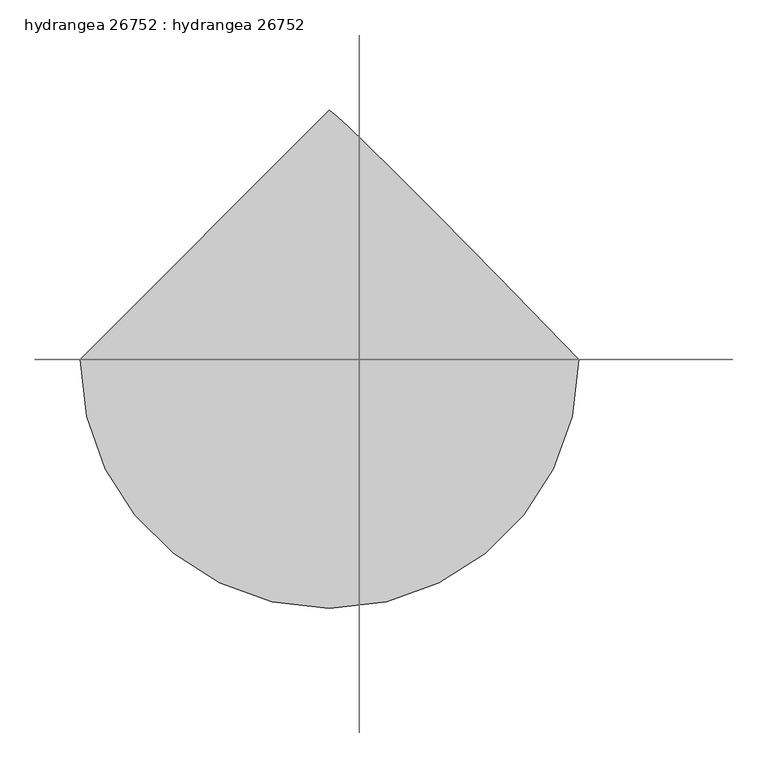
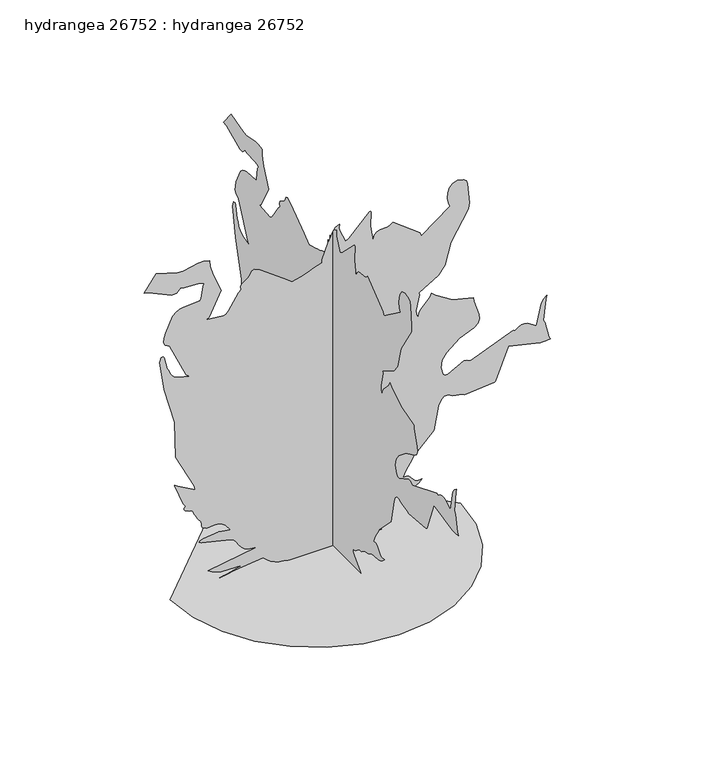
"""IFC4 building model written with IfcOpenShell, lengths in millimetres: proxy geometry, hydrangea 26752 : hydrangea 26752."""

from ifc_helpers import new_model, si_unit, origin, place, context, project, spatial, triangles, source, transform, mapped, element, save


def hydrangea_26752_hydrangea_26752_6cd4de68(model_context):
    return source(origin(), model_context, "Body", "Tessellation", [
        triangles([(-464.7672343, 0.0, 3.02e-05), (-452.4787039, -106.4936905, 3.02e-05), (-417.4875984, -204.2914365, 3.02e-05), (-362.5905132, -290.5916013, 3.02e-05), (-290.5916013, -362.5905132, 3.02e-05), (-204.2911822, -417.4875984, 3.02e-05), (-106.4936905, -452.4787039, 3.02e-05), (2.03e-05, -464.7672343, 3.02e-05), (106.4939449, -452.4787039, 3.02e-05), (204.2914365, -417.4875984, 3.02e-05), (290.5916013, -362.5905132, 3.02e-05), (362.5905132, -290.5916013, 3.02e-05), (417.4875984, -204.2911822, 3.02e-05), (452.4787039, -106.4936905, 3.02e-05), (464.7672343, 4.06e-05, 3.02e-05), (313.7284884, 154.9290062, 3.02e-05), (201.7549816, 268.9964805, 3.02e-05), (122.337727, 349.0116546, 3.02e-05), (68.9646404, 401.7878663, 3.02e-05), (35.1246865, 434.1297149, 3.02e-05), (14.3067201, 452.8546257, 3.02e-05), (-6.09e-05, 464.7672343, 3.02e-05), (56.0289111, -377.7746518, 894.66276), (56.0289111, -434.8662978, 988.0256659), (56.0289111, -437.025323, 1007.8783058), (56.0289111, -431.6938534, 1074.0784075), (56.0289111, -427.5688871, 1084.5381615), (56.0289111, -420.2181004, 1091.4545998), (56.0289111, -399.2732306, 1096.0341894), (56.0289111, -384.089092, 1091.3859993), (56.0289111, -374.1170626, 1079.9991943), (56.0289111, -368.8109911, 1064.3553091), (56.0289111, -367.6197121, 1046.9435812), (56.0289111, -369.9971832, 1030.2455452), (56.0289111, -375.3946735, 1016.7479679), (56.0289111, -283.8809099, 949.5141357), (56.0289111, -278.4503729, 960.8348837), (56.0289111, -192.0161139, 1027.487138), (56.0289111, -183.512436, 1019.3997683), (56.0289111, -173.3158381, 1016.575304), (56.0289111, -151.4921339, 1016.077442), (56.0289111, -141.6905156, 1013.0776978), (56.0289111, -133.8441922, 1004.6956512), (56.0289111, -128.8665527, 988.2669302), (56.0289111, -120.2805761, 1038.0128763), (56.0289111, -121.9587531, 1087.6699471), (56.0289111, -121.3283319, 1088.8815737), (56.0289111, -120.3204537, 1089.2625824), (56.0289111, -119.0941387, 1088.975536), (56.0289111, -117.8101691, 1088.1856133), (56.0289111, -51.0174846, 1022.5290831), (56.0289111, -40.1538944, 1015.3484894), (56.0289111, -21.3923125, 1059.6105406), (56.0289111, -19.9031842, 1068.9729778), (56.0289111, -20.5441289, 1080.248089), (56.0289111, -9.1964113, 1074.4568727), (56.0289111, -0.5405762, 1063.7304199), (56.0289111, 13.2029357, 1031.7950146), (56.0289111, 15.0194446, 1031.1828426), (56.0289111, 16.1084712, 1040.5605406), (56.0289111, 15.8290449, 1030.10333), (56.0289111, 34.9326629, 980.1719301), (56.0289111, 34.6535171, 969.7147923), (56.0289111, 46.9016657, 965.6583538), (56.0289111, 59.853396, 960.979715), (56.0289111, 73.3885619, 956.0013124), (56.0289111, 87.3888065, 951.0482718), (56.0289111, 101.7342336, 946.4457911), (56.0289111, 116.3062366, 942.5138363), (56.0289111, 130.9854187, 939.5776056), (56.0289111, 158.8299491, 961.2921232), (56.0289111, 234.3038488, 1015.5618484), (56.0289111, 252.5433605, 1023.7431805), (56.0289111, 260.6957517, 1020.4259411), (56.0289111, 264.4829115, 1008.7952557), (56.0289111, 270.9573709, 1001.4368385), (56.0289111, 292.1841821, 987.7081707), (56.0289111, 295.084859, 980.1414814), (56.0289111, 293.5100641, 968.1907574), (56.0289111, 301.5567932, 960.9593674), (56.0289111, 333.5786213, 911.8103325), (56.0289111, 341.9555446, 903.575588), (56.0289111, 350.6474195, 900.6063652), (56.0289111, 405.2778059, 906.5576008), (56.0289111, 397.091387, 912.3182957), (56.0289111, 357.3022459, 989.5521715), (56.0289111, 383.3829941, 1051.2462982), (56.0289111, 392.869915, 1083.2706516), (56.0289111, 394.0713315, 1102.6610378), (56.0289111, 413.8020676, 1107.4693199), (56.0289111, 431.2518745, 1106.8977705), (56.0289111, 479.0928497, 1096.097703), (56.0289111, 496.5959965, 1097.2025774), (56.0289111, 565.8923844, 1117.6013323), (56.0289111, 605.1150993, 1065.3077946), (56.0289111, 590.4389603, 1063.2046526), (56.0289111, 515.963528, 1028.2542423), (56.0289111, 499.8980115, 1030.0398165), (56.0289111, 487.4520052, 1042.8973166), (56.0289111, 476.9008324, 1039.305748), (56.0289111, 431.2823596, 1037.8351255), (56.0289111, 421.2823886, 1035.6633831), (56.0289111, 412.7479531, 1030.7561245), (56.0289111, 416.4106656, 1023.8879391), (56.0289111, 422.1561361, 984.398489), (56.0289111, 425.8213557, 977.5278328), (56.0289111, 478.1860737, 974.7465345), (56.0289111, 490.5939646, 971.7493338), (56.0289111, 502.2144762, 965.7473019), (56.0289111, 512.7834532, 955.7015488), (56.0289111, 536.4029417, 906.3493286), (56.0289111, 540.7590348, 890.4260273), (56.0289111, 541.4473649, 876.4001392), (56.0289111, 536.9465132, 865.9378418), (56.0289111, 523.4413055, 857.3729576), (56.0289111, 470.3247439, 742.9737631), (56.0289111, 459.1462111, 734.3275612), (56.0289111, 495.4784048, 743.0092987), (56.0289111, 506.2683349, 747.8099504), (56.0289111, 515.3336246, 754.7263887), (56.0289111, 522.0366674, 764.454574), (56.0289111, 525.7400024, 777.6930828), (56.0289111, 531.1476665, 784.7339321), (56.0289111, 539.8243172, 825.0565435), (56.0289111, 543.8298866, 829.879941), (56.0289111, 550.6015663, 829.2856459), (56.0289111, 555.6434461, 813.3064613), (56.0289111, 540.8123746, 716.5628025), (56.0289111, 507.4392663, 594.6655191), (56.0289111, 503.093347, 475.8365441), (56.0289111, 444.0484045, 359.0446904), (56.0289111, 441.1045435, 344.0002235), (56.0289111, 497.2995872, 374.7622267), (56.0289111, 506.1286268, 381.752316), (56.0289111, 507.3122755, 379.8777938), (56.0289111, 479.3442879, 309.3622215), (56.0289111, 471.5769931, 298.1760402), (56.0289111, 476.8474926, 293.4109968), (56.0289111, 476.8347754, 288.7729441), (56.0289111, 473.0577893, 284.5159002), (56.0289111, 460.289201, 278.1963731), (56.0289111, 454.3303714, 276.6495199), (56.0289111, 450.6829196, 276.5250544), (56.0289111, 447.9727289, 270.8405358), (56.0289111, 445.4428688, 265.374445), (56.0289111, 442.9105016, 259.9769365), (56.0289111, 440.1901734, 254.4981467), (56.0289111, 437.1015175, 248.789756), (56.0289111, 433.4642395, 242.6990667), (56.0289111, 429.0903422, 236.0780501), (56.0289111, 423.9341526, 231.4173971), (56.0289111, 421.2519035, 226.5421133), (56.0289111, 420.2282742, 221.6594716), (56.0289111, 420.0530305, 216.9764544), (56.0289111, 419.910779, 212.7001166), (56.0289111, 418.9912857, 209.0374223), (56.0289111, 416.4817732, 206.1956808), (56.0289111, 404.3481751, 201.1304013), (56.0289111, 392.979138, 200.8065475), (56.0289111, 381.7802576, 202.325223), (56.0289111, 370.1622894, 202.7872406), (56.0289111, 357.5257424, 199.293722), (56.0289111, 343.2814084, 188.9454982), (56.0289111, 326.8374267, 168.843146), (56.0289111, 363.7335394, 174.8182537), (56.0289111, 415.2447847, 168.959745), (56.0289111, 424.7621907, 165.1799612), (56.0289111, 427.6882476, 161.3724901), (56.0289111, 422.6031655, 158.3819023), (56.0289111, 326.8374267, 135.2257031), (56.0289111, 316.3675352, 128.5444794), (56.0289111, 308.4071926, 119.1548454), (56.0289111, 301.2011826, 108.4708318), (56.0289111, 292.9842786, 97.9059425), (56.0289111, 281.9936886, 88.8741991), (56.0289111, 266.4742689, 82.7891145), (56.0289111, 244.6604659, 81.0642016), (56.0289111, 399.6745505, 54.9174055), (56.0289111, 387.1320385, 46.4490362), (56.0289111, 358.6535079, 37.4287247), (56.0289111, 291.3510571, 36.2410178), (56.0289111, 337.9144032, 23.9287606), (56.0289111, 349.4180614, 21.3156048), (56.0289111, 362.3212709, 18.4984871), (56.0289111, 355.630909, 19.454849), (56.0289111, 338.5316257, 22.4599004), (56.0289111, 314.6454383, 26.6484415), (56.0289111, 223.7308386, 37.9362155), (56.0289111, 211.5466986, 26.1533955), (56.0289111, 198.7755668, 17.3074794), (56.0289111, 185.515475, 10.9090339), (56.0289111, 171.8642371, 6.4684733), (56.0289111, 157.9193579, 3.4965937), (56.0289111, 143.7791599, 1.5035523), (56.0289111, 129.5409211, 0.0), (56.0289111, -156.3006158, 8.5e-06), (56.0289111, -151.6640893, 6.8894283), (56.0289111, -116.3057279, 38.9204668), (56.0289111, -111.4957199, 47.331436), (56.0289111, -111.590972, 55.6176853), (56.0289111, -119.3379828, 56.8782915), (56.0289111, -125.2241879, 59.5351333), (56.0289111, -130.2038621, 63.1188217), (56.0289111, -135.2315439, 67.1597133), (56.0289111, -141.2622714, 71.1881602), (56.0289111, -149.2498198, 74.7345099), (56.0289111, -160.1494906, 77.329128), (56.0289111, -168.9650681, 83.9521794), (56.0289111, -176.5355544, 87.5539036), (56.0289111, -196.7577757, 92.3169214), (56.0289111, -204.3280077, 95.9186456), (56.0289111, -213.1436033, 102.5419604), (56.0289111, -254.4092531, 106.5686224), (56.0289111, -265.3388912, 110.053257), (56.0289111, -275.7884532, 116.2788036), (56.0289111, -285.3972962, 126.1210626), (56.0289111, -270.7287694, 125.7187253), (56.0289111, -261.0386631, 129.5500684), (56.0289111, -244.0602664, 149.2523633), (56.0289111, -236.5088377, 152.8248832), (56.0289111, -225.0498715, 152.0344246), (56.0289111, -234.5898597, 172.6625532), (56.0289111, -246.2180017, 193.2690897), (56.0289111, -259.5756166, 213.3033683), (56.0289111, -323.1010995, 276.6977727), (56.0289111, -338.0566183, 354.6326777), (56.0289111, -345.6055398, 371.0131823), (56.0289111, -356.2354506, 380.7922002), (56.0289111, -370.7261358, 381.2874825), (56.0289111, -376.1719153, 376.5935466), (56.0289111, -382.951189, 373.9163844), (56.0289111, -414.431971, 368.0820022), (56.0289111, -421.1503109, 364.0103757), (56.0289111, -516.6848866, 372.087608), (56.0289111, -521.0689213, 374.2821688), (56.0289111, -561.6327971, 477.6729873), (56.0289111, -663.3141632, 454.759633), (56.0289111, -683.0017696, 454.2617709), (56.0289111, -696.6263014, 456.4588752), (56.0289111, -691.4650612, 464.9628256), (56.0289111, -679.3771362, 518.9251568), (56.0289111, -674.215896, 527.4291072), (56.0289111, -681.6479279, 594.9220805), (56.0289111, -685.4224068, 606.8042041), (56.0289111, -674.9575659, 597.7338638), (56.0289111, -667.4314991, 587.1039531), (56.0289111, -651.805418, 516.2225965), (56.0289111, -623.5224787, 533.9975653), (56.0289111, -613.96703, 536.3114865), (56.0289111, -604.0863831, 535.7831758), (56.0289111, -593.7181206, 531.7852003), (56.0289111, -582.7021142, 523.6927437), (56.0289111, -577.4646432, 527.2970295), (56.0289111, -440.4085831, 471.9960809), (56.0289111, -429.7609045, 477.805065), (56.0289111, -420.0225454, 479.0471403), (56.0289111, -367.9321567, 451.6074635), (56.0289111, -358.5290606, 450.3882792), (56.0289111, -353.3322121, 456.9262522), (56.0289111, -345.7960078, 481.3356634), (56.0289111, -350.0683125, 504.1753667), (56.0289111, -363.3880663, 525.0059266), (56.0289111, -406.1337856, 558.9200629), (56.0289111, -451.9579871, 579.6160017), (56.0289111, -465.1685543, 589.0190978), (56.0289111, -469.6389573, 603.0043633), (56.0289111, -467.9142806, 619.826774), (56.0289111, -451.0918336, 669.8597666), (56.0289111, -450.0987256, 680.5760456), (56.0289111, -383.0096157, 698.4017744), (56.0289111, -329.3240845, 731.7240864), (56.0289111, -316.5631265, 743.6087534), (56.0289111, -311.5136164, 731.6199503), (56.0289111, -280.6932047, 700.0375757), (56.0289111, -275.2499687, 690.0807707), (56.0289111, -272.6744173, 676.8397184), (56.0289111, -266.9721128, 689.0418806), (56.0289111, -265.8748323, 702.5623489), (56.0289111, -277.0838502, 752.2879475), (56.0289111, -276.1770741, 759.2500952), (56.0289111, -338.0413939, 796.367161), (56.0289111, -358.8363819, 823.4360029), (433.8020459, 5.25e-05, 894.66276), (490.8936919, 6.21e-05, 988.0256659), (493.0552242, 6.39e-05, 1007.8783058), (487.7237909, 6.93e-05, 1074.0784075), (483.5988247, 7.01e-05, 1084.5381615), (476.2454945, 7.04e-05, 1091.4545998), (455.3006247, 7.02e-05, 1096.0341894), (440.1164861, 6.93e-05, 1091.3859993), (430.1470001, 6.81e-05, 1079.9991943), (424.8383852, 6.66e-05, 1064.3553091), (423.6496496, 6.51e-05, 1046.9435812), (426.0270844, 6.37e-05, 1030.2455452), (431.4246111, 6.27e-05, 1016.7479679), (339.9082858, 5.44e-05, 949.5141357), (334.477767, 5.52e-05, 960.8348837), (248.0447615, 5.82e-05, 1027.487138), (239.541338, 5.73e-05, 1019.3997683), (229.3447583, 5.67e-05, 1016.575304), (207.5210541, 5.6e-05, 1016.077442), (197.7191814, 5.55e-05, 1013.0776978), (189.8731124, 5.45e-05, 1004.6956512), (184.8952004, 5.3e-05, 988.2669302), (176.3092419, 5.66e-05, 1038.0128763), (177.9874098, 6.11e-05, 1087.6699471), (177.3572339, 6.11e-05, 1088.8815737), (176.3491196, 6.1e-05, 1089.2625824), (175.1227954, 6.09e-05, 1088.975536), (173.8390802, 6.07e-05, 1088.1856133), (107.0464002, 5.35e-05, 1022.5290831), (96.182801, 5.27e-05, 1015.3484894), (77.4210737, 5.59e-05, 1059.6105406), (75.9321248, 5.66e-05, 1068.9729778), (76.5729696, 5.75e-05, 1080.248089), (65.2252475, 5.67e-05, 1074.4568727), (56.5694259, 5.55e-05, 1063.7304199), (42.8259742, 5.23e-05, 1031.7950146), (41.0093655, 5.23e-05, 1031.1828426), (39.9204648, 5.31e-05, 1040.5605406), (40.1998673, 5.22e-05, 1030.10333), (21.0960983, 4.75e-05, 980.1719301), (21.3753963, 4.66e-05, 969.7147923), (9.1270438, 4.59e-05, 965.6583538), (-3.8244574, 4.51e-05, 960.979715), (-17.3597019, 4.43e-05, 956.0013124), (-31.3598954, 4.34e-05, 951.0482718), (-45.7053225, 4.26e-05, 946.4457911), (-60.2773209, 4.18e-05, 942.5138363), (-74.9565076, 4.11e-05, 939.5776056), (-102.801038, 4.21e-05, 961.2921232), (-178.2749468, 4.45e-05, 1015.5618484), (-196.5144585, 4.46e-05, 1023.7431805), (-204.6668497, 4.41e-05, 1020.4259411), (-208.4534826, 4.3e-05, 1008.7952557), (-214.9284508, 4.22e-05, 1001.4368385), (-236.1547533, 4.05e-05, 987.7081707), (-239.055957, 3.97e-05, 980.1414814), (-237.481907, 3.88e-05, 968.1907574), (-245.5273643, 3.79e-05, 960.9593674), (-277.5486837, 3.28e-05, 911.8103325), (-285.9281505, 3.19e-05, 903.575588), (-294.6200436, 3.14e-05, 900.6063652), (-349.2479047, 3.02e-05, 906.5576008), (-341.0639929, 3.09e-05, 912.3182957), (-301.2723083, 3.86e-05, 989.5521715), (-327.3530565, 4.31e-05, 1051.2462982), (-336.8399775, 4.55e-05, 1083.2706516), (-338.0413939, 4.71e-05, 1102.6610378), (-357.77213, 4.69e-05, 1107.4693199), (-375.2244804, 4.63e-05, 1106.8977705), (-423.0654556, 4.4e-05, 1096.097703), (-440.5660953, 4.36e-05, 1097.2025774), (-509.8649903, 4.32e-05, 1117.6013323), (-549.0851618, 3.76e-05, 1065.3077946), (-534.4115662, 3.79e-05, 1063.2046526), (-459.9361339, 3.72e-05, 1028.2542423), (-443.8706174, 3.78e-05, 1030.0398165), (-431.4246111, 3.93e-05, 1042.8973166), (-420.8734383, 3.93e-05, 1039.305748), (-375.252422, 4.05e-05, 1037.8351255), (-365.252451, 4.06e-05, 1035.6633831), (-356.7180519, 4.05e-05, 1030.7561245), (-360.3832715, 3.98e-05, 1023.8879391), (-366.128742, 3.63e-05, 984.398489), (-369.7914182, 3.56e-05, 977.5278328), (-422.1586796, 3.38e-05, 974.7465345), (-434.5666068, 3.32e-05, 971.7493338), (-446.184575, 3.23e-05, 965.7473019), (-456.7535156, 3.12e-05, 955.7015488), (-480.3730042, 2.63e-05, 906.3493286), (-484.7290973, 2.48e-05, 890.4260273), (-485.4174637, 2.36e-05, 876.4001392), (-480.9165756, 2.29e-05, 865.9378418), (-467.4139114, 2.25e-05, 857.3729576), (-414.2948427, 1.45e-05, 742.9737631), (-403.118817, 1.41e-05, 734.3275612), (-439.4484673, 1.37e-05, 743.0092987), (-450.2383973, 1.38e-05, 747.8099504), (-459.303687, 1.42e-05, 754.7263887), (-466.0067662, 1.48e-05, 764.454574), (-469.7100649, 1.58e-05, 777.6930828), (-475.117729, 1.62e-05, 784.7339321), (-483.7943796, 1.93e-05, 825.0565435), (-487.7999854, 1.96e-05, 829.879941), (-494.5741722, 1.93e-05, 829.2856459), (-499.6160883, 1.78e-05, 813.3064613), (-484.782437, 1.01e-05, 716.5628025), (-451.4119085, 9e-07, 594.6655191), (-447.0659529, -9e-06, 475.8365441), (-388.0210467, -1.71e-05, 359.0446904), (-385.0746423, -1.83e-05, 344.0002235), (-441.2721931, -1.73e-05, 374.7622267), (-450.1012327, -1.7e-05, 381.752316), (-451.2848814, -1.73e-05, 379.8777938), (-423.3143867, -2.24e-05, 309.3622215), (-415.549599, -2.3e-05, 298.1760402), (-420.817555, -2.36e-05, 293.4109968), (-420.8048378, -2.39e-05, 288.7729441), (-417.0303952, -2.41e-05, 284.5159002), (-404.2592634, -2.42e-05, 278.1963731), (-398.3029773, -2.42e-05, 276.6495199), (-394.6555255, -2.42e-05, 276.5250544), (-391.9453348, -2.46e-05, 270.8405358), (-389.4129676, -2.5e-05, 265.374445), (-386.880564, -2.54e-05, 259.9769365), (-384.1602359, -2.58e-05, 254.4981467), (-381.0741234, -2.62e-05, 248.789756), (-377.4343019, -2.65e-05, 242.6990667), (-373.0604047, -2.7e-05, 236.0780501), (-367.9067585, -2.72e-05, 231.4173971), (-365.221966, -2.76e-05, 226.5421133), (-364.1983366, -2.8e-05, 221.6594716), (-364.0230929, -2.84e-05, 216.9764544), (-363.8808414, -2.87e-05, 212.7001166), (-362.9613482, -2.9e-05, 209.0374223), (-360.4543791, -2.92e-05, 206.1956808), (-348.320781, -2.92e-05, 201.1304013), (-336.9492004, -2.89e-05, 200.8065475), (-325.7528635, -2.84e-05, 202.325223), (-314.1323519, -2.81e-05, 202.7872406), (-301.4983665, -2.8e-05, 199.293722), (-287.2540325, -2.84e-05, 188.9454982), (-270.8075073, -2.96e-05, 168.843146), (-307.7036018, -3e-05, 174.8182537), (-359.2173906, -3.17e-05, 168.959745), (-368.7322532, -3.24e-05, 165.1799612), (-371.6583464, -3.32e-05, 161.3724901), (-366.5732643, -3.31e-05, 158.3819023), (-270.8075073, -3.24e-05, 135.2257031), (-260.3376158, -3.27e-05, 128.5444794), (-252.3792717, -3.32e-05, 119.1548454), (-245.1717719, -3.39e-05, 108.4708318), (-236.9543411, -3.46e-05, 97.9059425), (-225.9652771, -3.51e-05, 88.8741991), (-210.44484, -3.51e-05, 82.7891145), (-188.6315457, -3.46e-05, 81.0642016), (-343.6446493, -4.14e-05, 54.9174055), (-331.1021009, -4.15e-05, 46.4490362), (-302.6235885, -4.14e-05, 37.4287247), (-235.3221369, -3.98e-05, 36.2410178), (-281.887009, -4.21e-05, 23.9287856), (-293.3906855, -4.27e-05, 21.3156298), (-306.2913697, -4.33e-05, 18.498512), (-299.6009896, -4.31e-05, 19.454874), (-282.5016881, -4.23e-05, 22.4599277), (-258.6180442, -4.13e-05, 26.6484415), (-167.7021728, -3.76e-05, 37.9362155), (-155.5177784, -3.82e-05, 26.1533955), (-142.7466466, -3.86e-05, 17.3074794), (-129.4865639, -3.88e-05, 10.9090589), (-115.8353169, -3.87e-05, 6.4684733), (-101.8904468, -3.85e-05, 3.496619), (-87.7502488, -3.83e-05, 1.5035625), (-73.5122598, -3.8e-05, 9.2e-06), (212.3292817, -2.95e-05, 5.3e-06), (207.6930094, -2.9e-05, 6.8894283), (172.3346299, -2.74e-05, 38.9204668), (167.52464, -2.68e-05, 47.331436), (167.6196379, -2.61e-05, 55.6176853), (175.3668939, -2.58e-05, 56.8782915), (181.2528355, -2.54e-05, 59.5351333), (186.2325279, -2.49e-05, 63.1188217), (191.2602007, -2.44e-05, 67.1597133), (197.2911916, -2.39e-05, 71.1881602), (205.2787309, -2.34e-05, 74.7345099), (216.1781383, -2.29e-05, 77.329128), (224.9937339, -2.2e-05, 83.9521794), (232.5642021, -2.15e-05, 87.5539036), (252.7864416, -2.05e-05, 92.3169214), (260.3579453, -2e-05, 95.9186456), (269.1717423, -1.91e-05, 102.5419604), (310.4366472, -1.75e-05, 106.5686224), (321.3688288, -1.69e-05, 110.0530027), (331.8183726, -1.61e-05, 116.2788036), (341.4272338, -1.5e-05, 126.1210626), (326.7586887, -1.55e-05, 125.7187253), (317.0660391, -1.54e-05, 129.5500684), (300.0886597, -1.43e-05, 149.2523633), (292.5372311, -1.42e-05, 152.8248832), (281.0792822, -1.46e-05, 152.0344246), (290.6195429, -1.26e-05, 172.6625532), (302.2476667, -1.05e-05, 193.2690897), (315.6030107, -8.4e-06, 213.3033683), (379.1284936, -1.2e-06, 276.6977727), (394.0840124, 5.8e-06, 354.6326777), (401.6328976, 7.5e-06, 371.0131823), (412.2628083, 8.6e-06, 380.7922002), (426.7535299, 9.1e-06, 381.2874825), (432.1993094, 8.8e-06, 376.5935466), (438.9785831, 8.8e-06, 373.9163844), (470.4619085, 9.3e-06, 368.0820022), (477.1802121, 9.1e-06, 364.0103757), (572.7148241, 1.25e-05, 372.087608), (577.0988588, 1.3e-05, 374.2821688), (617.6601912, 2.29e-05, 477.6729873), (719.3415573, 2.4e-05, 454.759633), (739.0291637, 2.45e-05, 454.2617709), (752.6562389, 2.51e-05, 456.4588752), (747.4949987, 2.57e-05, 464.9628256), (735.4070738, 2.99e-05, 518.9251568), (730.2458336, 3.04e-05, 527.4291072), (737.6778654, 3.63e-05, 594.9220805), (741.4498009, 3.74e-05, 606.8042041), (730.9875034, 3.64e-05, 597.7338638), (723.4614367, 3.53e-05, 587.1039531), (707.8328121, 2.88e-05, 516.2225965), (679.5498728, 2.95e-05, 533.9975653), (669.9969675, 2.94e-05, 536.3114865), (660.1163206, 2.91e-05, 535.7831758), (649.7455147, 2.84e-05, 531.7852003), (638.729472, 2.74e-05, 523.6927437), (633.492001, 2.76e-05, 527.2970295), (496.4359772, 1.88e-05, 471.9960809), (485.7882986, 1.9e-05, 477.805065), (476.0524467, 1.88e-05, 479.0471403), (423.9620942, 1.49e-05, 451.6074635), (414.5564547, 1.45e-05, 450.3882792), (409.3621496, 1.49e-05, 456.9262522), (401.8259454, 1.72e-05, 481.3356634), (406.09825, 1.94e-05, 504.1753667), (419.4180038, 2.15e-05, 525.0059266), (462.1637232, 2.53e-05, 558.9200629), (507.9853812, 2.82e-05, 579.6160017), (521.1984919, 2.94e-05, 589.0190978), (525.6663514, 3.07e-05, 603.0043633), (523.9442182, 3.21e-05, 619.826774), (507.1192277, 3.58e-05, 669.8597666), (506.1286268, 3.66e-05, 680.5760456), (439.0370098, 3.62e-05, 698.4017744), (385.3514786, 3.74e-05, 731.7240864), (372.593064, 3.8e-05, 743.6087534), (367.5409741, 3.68e-05, 731.6199503), (336.7231241, 3.32e-05, 700.0375757), (331.2773809, 3.22e-05, 690.0807707), (328.7043549, 3.11e-05, 676.8397184), (323.0020503, 3.19e-05, 689.0418806), (321.9022264, 3.3e-05, 702.5623489), (333.1112443, 3.76e-05, 752.2879475), (332.2044683, 3.81e-05, 759.2500952), (394.0713315, 4.31e-05, 796.367161), (414.8663195, 4.6e-05, 823.4360029)], [[21, 22, 1], [20, 21, 1], [19, 20, 1], [18, 19, 1], [17, 18, 1], [17, 1, 2], [17, 2, 3], [17, 3, 4], [16, 17, 4], [16, 4, 5], [16, 5, 6], [16, 6, 7], [16, 7, 8], [16, 8, 9], [16, 9, 10], [16, 10, 11], [16, 11, 12], [15, 16, 12], [14, 15, 12], [13, 14, 12], [183, 184, 185], [59, 60, 61], [183, 185, 186], [182, 183, 186], [243, 244, 245], [177, 178, 179], [215, 216, 217], [195, 196, 197], [195, 197, 198], [182, 186, 187], [181, 182, 187], [181, 187, 188], [54, 55, 56], [94, 95, 96], [238, 239, 240], [195, 198, 199], [271, 272, 273], [167, 168, 169], [133, 134, 135], [214, 215, 217], [214, 217, 218], [177, 179, 180], [177, 180, 181], [166, 167, 169], [165, 166, 169], [164, 165, 169], [164, 169, 170], [37, 38, 39], [213, 214, 218], [94, 96, 97], [93, 94, 97], [93, 97, 98], [93, 98, 99], [92, 93, 99], [92, 99, 100], [92, 100, 101], [91, 92, 101], [90, 91, 101], [90, 101, 102], [89, 90, 102], [88, 89, 102], [87, 88, 102], [87, 102, 103], [195, 199, 200], [54, 56, 57], [53, 54, 57], [243, 245, 246], [242, 243, 246], [242, 246, 247], [241, 242, 247], [268, 269, 270], [87, 103, 104], [86, 87, 104], [86, 104, 105], [86, 105, 106], [85, 86, 106], [84, 85, 106], [133, 135, 136], [132, 133, 136], [132, 136, 137], [53, 57, 58], [125, 126, 127], [124, 125, 127], [123, 124, 127], [123, 127, 128], [122, 123, 128], [121, 122, 128], [120, 121, 128], [119, 120, 128], [52, 53, 58], [177, 181, 188], [118, 119, 128], [213, 218, 219], [213, 219, 220], [213, 220, 221], [212, 213, 221], [117, 118, 128], [164, 170, 171], [237, 238, 240], [237, 240, 241], [237, 241, 247], [237, 247, 248], [237, 248, 249], [237, 249, 250], [237, 250, 251], [237, 251, 252], [236, 237, 252], [236, 252, 253], [236, 253, 254], [235, 236, 254], [234, 235, 254], [233, 234, 254], [232, 233, 254], [232, 254, 255], [232, 255, 256], [232, 256, 257], [231, 232, 257], [230, 231, 257], [229, 230, 257], [229, 257, 258], [228, 229, 258], [84, 106, 107], [84, 107, 108], [84, 108, 109], [84, 109, 110], [84, 110, 111], [84, 111, 112], [84, 112, 113], [84, 113, 114], [84, 114, 115], [84, 115, 116], [84, 116, 117], [83, 84, 117], [270, 271, 273], [73, 74, 75], [72, 73, 75], [137, 138, 139], [137, 139, 140], [137, 140, 141], [132, 137, 141], [132, 141, 142], [132, 142, 143], [72, 75, 76], [227, 228, 258], [227, 258, 259], [117, 128, 129], [224, 225, 226], [46, 47, 48], [46, 48, 49], [46, 49, 50], [45, 46, 50], [45, 50, 51], [44, 45, 51], [44, 51, 52], [211, 212, 221], [210, 211, 221], [209, 210, 221], [82, 83, 117], [270, 273, 274], [270, 274, 275], [270, 275, 276], [264, 265, 266], [264, 266, 267], [264, 267, 268], [264, 268, 270], [263, 264, 270], [263, 270, 276], [262, 263, 276], [261, 262, 276], [52, 58, 59], [52, 59, 61], [52, 61, 62], [52, 62, 63], [44, 52, 63], [260, 261, 276], [71, 72, 76], [71, 76, 77], [71, 77, 78], [71, 78, 79], [71, 79, 80], [70, 71, 80], [70, 80, 81], [70, 81, 82], [70, 82, 117], [70, 117, 129], [70, 129, 130], [70, 130, 131], [69, 70, 131], [68, 69, 131], [67, 68, 131], [67, 131, 132], [66, 67, 132], [65, 66, 132], [64, 65, 132], [63, 64, 132], [44, 63, 132], [132, 143, 144], [44, 132, 144], [44, 144, 145], [44, 145, 146], [44, 146, 147], [44, 147, 148], [44, 148, 149], [44, 149, 150], [44, 150, 151], [44, 151, 152], [44, 152, 153], [44, 153, 154], [44, 154, 155], [44, 155, 156], [44, 156, 157], [44, 157, 158], [44, 158, 159], [44, 159, 160], [44, 160, 161], [44, 161, 162], [44, 162, 163], [44, 163, 164], [44, 164, 171], [44, 171, 172], [44, 172, 173], [44, 173, 174], [44, 174, 175], [44, 175, 176], [44, 176, 177], [44, 177, 188], [44, 188, 189], [44, 189, 190], [44, 190, 191], [44, 191, 192], [44, 192, 193], [44, 193, 194], [44, 194, 195], [44, 195, 200], [44, 200, 201], [44, 201, 202], [44, 202, 203], [44, 203, 204], [44, 204, 205], [44, 205, 206], [44, 206, 207], [44, 207, 208], [44, 208, 209], [44, 209, 221], [44, 221, 222], [44, 222, 223], [44, 223, 224], [44, 224, 226], [44, 226, 227], [44, 227, 259], [44, 259, 260], [43, 44, 260], [42, 43, 260], [29, 30, 31], [28, 29, 31], [28, 31, 32], [27, 28, 32], [26, 27, 32], [26, 32, 33], [26, 33, 34], [26, 34, 35], [25, 26, 35], [24, 25, 35], [23, 24, 35], [23, 35, 36], [282, 23, 36], [281, 282, 36], [280, 281, 36], [37, 39, 40], [280, 36, 37], [280, 37, 40], [280, 40, 41], [280, 41, 42], [279, 280, 42], [278, 279, 42], [277, 278, 42], [277, 42, 260], [277, 260, 276], [443, 444, 445], [319, 320, 321], [443, 445, 446], [442, 443, 446], [503, 504, 505], [437, 438, 439], [475, 476, 477], [455, 456, 457], [455, 457, 458], [442, 446, 447], [441, 442, 447], [441, 447, 448], [314, 315, 316], [354, 355, 356], [498, 499, 500], [455, 458, 459], [531, 532, 533], [427, 428, 429], [393, 394, 395], [474, 475, 477], [474, 477, 478], [437, 439, 440], [437, 440, 441], [426, 427, 429], [425, 426, 429], [424, 425, 429], [424, 429, 430], [297, 298, 299], [473, 474, 478], [354, 356, 357], [353, 354, 357], [353, 357, 358], [353, 358, 359], [352, 353, 359], [352, 359, 360], [352, 360, 361], [351, 352, 361], [350, 351, 361], [350, 361, 362], [349, 350, 362], [348, 349, 362], [347, 348, 362], [347, 362, 363], [455, 459, 460], [314, 316, 317], [313, 314, 317], [503, 505, 506], [502, 503, 506], [502, 506, 507], [501, 502, 507], [528, 529, 530], [347, 363, 364], [346, 347, 364], [346, 364, 365], [346, 365, 366], [345, 346, 366], [344, 345, 366], [393, 395, 396], [392, 393, 396], [392, 396, 397], [313, 317, 318], [385, 386, 387], [384, 385, 387], [383, 384, 387], [383, 387, 388], [382, 383, 388], [381, 382, 388], [380, 381, 388], [379, 380, 388], [312, 313, 318], [437, 441, 448], [378, 379, 388], [473, 478, 479], [473, 479, 480], [473, 480, 481], [472, 473, 481], [377, 378, 388], [424, 430, 431], [497, 498, 500], [497, 500, 501], [497, 501, 507], [497, 507, 508], [497, 508, 509], [497, 509, 510], [497, 510, 511], [497, 511, 512], [496, 497, 512], [496, 512, 513], [496, 513, 514], [495, 496, 514], [494, 495, 514], [493, 494, 514], [492, 493, 514], [492, 514, 515], [492, 515, 516], [492, 516, 517], [491, 492, 517], [490, 491, 517], [489, 490, 517], [489, 517, 518], [488, 489, 518], [344, 366, 367], [344, 367, 368], [344, 368, 369], [344, 369, 370], [344, 370, 371], [344, 371, 372], [344, 372, 373], [344, 373, 374], [344, 374, 375], [344, 375, 376], [344, 376, 377], [343, 344, 377], [530, 531, 533], [333, 334, 335], [332, 333, 335], [397, 398, 399], [397, 399, 400], [397, 400, 401], [392, 397, 401], [392, 401, 402], [392, 402, 403], [332, 335, 336], [487, 488, 518], [487, 518, 519], [377, 388, 389], [484, 485, 486], [306, 307, 308], [306, 308, 309], [306, 309, 310], [305, 306, 310], [305, 310, 311], [304, 305, 311], [304, 311, 312], [471, 472, 481], [470, 471, 481], [469, 470, 481], [342, 343, 377], [530, 533, 534], [530, 534, 535], [530, 535, 536], [524, 525, 526], [524, 526, 527], [524, 527, 528], [524, 528, 530], [523, 524, 530], [523, 530, 536], [522, 523, 536], [521, 522, 536], [312, 318, 319], [312, 319, 321], [312, 321, 322], [312, 322, 323], [304, 312, 323], [520, 521, 536], [331, 332, 336], [331, 336, 337], [331, 337, 338], [331, 338, 339], [331, 339, 340], [330, 331, 340], [330, 340, 341], [330, 341, 342], [330, 342, 377], [330, 377, 389], [330, 389, 390], [330, 390, 391], [329, 330, 391], [328, 329, 391], [327, 328, 391], [327, 391, 392], [326, 327, 392], [325, 326, 392], [324, 325, 392], [323, 324, 392], [304, 323, 392], [392, 403, 404], [304, 392, 404], [304, 404, 405], [304, 405, 406], [304, 406, 407], [304, 407, 408], [304, 408, 409], [304, 409, 410], [304, 410, 411], [304, 411, 412], [304, 412, 413], [304, 413, 414], [304, 414, 415], [304, 415, 416], [304, 416, 417], [304, 417, 418], [304, 418, 419], [304, 419, 420], [304, 420, 421], [304, 421, 422], [304, 422, 423], [304, 423, 424], [304, 424, 431], [304, 431, 432], [304, 432, 433], [304, 433, 434], [304, 434, 435], [304, 435, 436], [304, 436, 437], [304, 437, 448], [304, 448, 449], [304, 449, 450], [304, 450, 451], [304, 451, 452], [304, 452, 453], [304, 453, 454], [304, 454, 455], [304, 455, 460], [304, 460, 461], [304, 461, 462], [304, 462, 463], [304, 463, 464], [304, 464, 465], [304, 465, 466], [304, 466, 467], [304, 467, 468], [304, 468, 469], [304, 469, 481], [304, 481, 482], [304, 482, 483], [304, 483, 484], [304, 484, 486], [304, 486, 487], [304, 487, 519], [304, 519, 520], [303, 304, 520], [302, 303, 520], [289, 290, 291], [288, 289, 291], [288, 291, 292], [287, 288, 292], [286, 287, 292], [286, 292, 293], [286, 293, 294], [286, 294, 295], [285, 286, 295], [284, 285, 295], [283, 284, 295], [283, 295, 296], [542, 283, 296], [541, 542, 296], [540, 541, 296], [297, 299, 300], [540, 296, 297], [540, 297, 300], [540, 300, 301], [540, 301, 302], [539, 540, 302], [538, 539, 302], [537, 538, 302], [537, 302, 520], [537, 520, 536]], closed=False),
    ])


if __name__ == "__main__":
    model = new_model("IFC4")
    model_context = context("Model", 3, world=origin())
    ifc_project = project(units=[si_unit("LENGTHUNIT", "METRE", prefix="MILLI")], contexts=[model_context])
    site = spatial("IfcSite", under=ifc_project)
    building = spatial("IfcBuilding", under=site)
    placement = place(None, origin())
    hydrangea_26752_hydrangea_26752_shape = hydrangea_26752_hydrangea_26752_6cd4de68(model_context)
    element("IfcBuildingElementProxy", 1, Name="hydrangea 26752 : hydrangea 26752", ObjectType="hydrangea 26752 : hydrangea 26752", at=placement, inside=building, context=model_context, shape_type="MappedRepresentation", body=[
        mapped(hydrangea_26752_hydrangea_26752_shape, transform((0.0, 0.0, 0.0), x_axis=(1.0, 0.0, 0.0), y_axis=(0.0, 1.0, 0.0), z_axis=(0.0, 0.0, 1.0))),
    ])
    save(model, "model.ifc")

# Revit data of these elements
# Type "hydrangea 26752 : hydrangea 26752"
#   built-in parameter 1005195 = "RPC-16-FW46-UP80-R12G-Q000-ST1L-LVER-AU"
#   Height = 0
